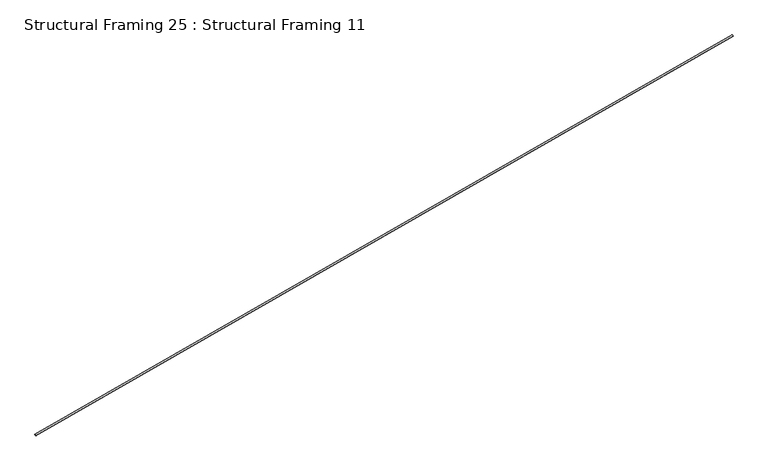
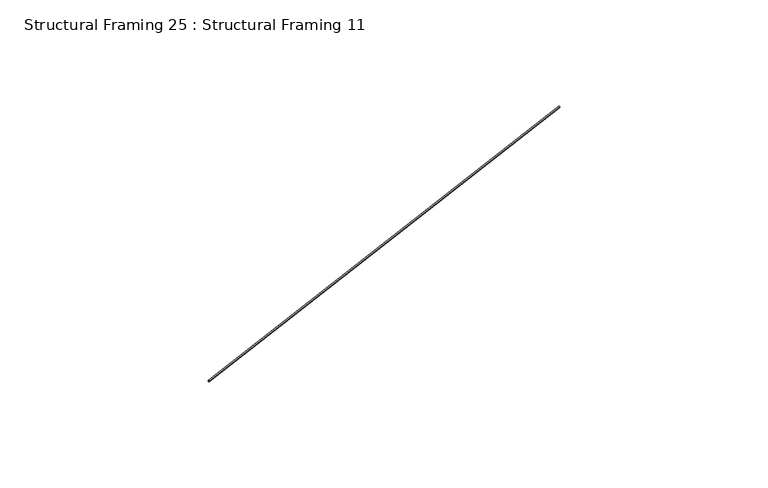
"""IFC4 building model written with IfcOpenShell, lengths in millimetres: beam geometry, Structural Framing 25 : Structural Framing 11."""

from ifc_helpers import new_model, si_unit, point, frame, origin, origin_2d, place, context, project, spatial, circle_curve, trimmed, segment, composite_curve, outline, extrude, source, transform, mapped, element, save


def structural_framing_25_structural_framing_11_07be0c14(model_context):
    return source(origin(), model_context, "Body", "SweptSolid", [
        extrude(outline(composite_curve([segment(trimmed(circle_curve(origin_2d(), 6.35), [point((0.0, 6.35))], [point((0.0, -6.35))], False, "CARTESIAN"), True, "CONTINUOUS"), segment(trimmed(circle_curve(origin_2d(), 6.35), [point((0.0, -6.35))], [point((0.0, 6.35))], False, "CARTESIAN"), True, "CONTINUOUS")], self_intersect=False)), frame((28346.1075052, 10045.6198795, 4934.1500933), z_axis=(-0.8608596592499242, -0.49364969439624967, 0.12341242359905893), x_axis=(0.0, 0.24253562503632659, 0.9701425001453335)), (0.0, 0.0, 1.0), 5892.4476777),
    ])


if __name__ == "__main__":
    model = new_model("IFC4")
    model_context = context("Model", 3, world=origin())
    ifc_project = project(units=[si_unit("LENGTHUNIT", "METRE", prefix="MILLI")], contexts=[model_context])
    site = spatial("IfcSite", under=ifc_project)
    building = spatial("IfcBuilding", under=site)
    placement = place(None, origin())
    structural_framing_25_structural_framing_11_shape = structural_framing_25_structural_framing_11_07be0c14(model_context)
    element("IfcBeam", 1, ObjectType="Structural Framing 25 : Structural Framing 11", at=placement, inside=building, context=model_context, shape_type="MappedRepresentation", body=[
        mapped(structural_framing_25_structural_framing_11_shape, transform((0.0, 0.0, 0.0), x_axis=(1.0, 0.0, 0.0), y_axis=(0.0, 1.0, 0.0), z_axis=(0.0, 0.0, 1.0))),
    ])
    save(model, "model.ifc")

# Revit data of these elements
# Type "Structural Framing 25 : Structural Framing 11"
#   Structural Material [instance default] = EXISTING LATERAL BRACING (1/4" CABLE)
# Element 1 (IfcBeam, "Structural Framing 25 : Structural Framing 11")
#   Materials on its faces: "EXISTING LATERAL BRACING (1/4\" CABLE)"
# Materials
#   "EXISTING LATERAL BRACING (1/4\" CABLE)": class "Generic", colour RGB 120 120 120, transparency 0, Cost = 0
